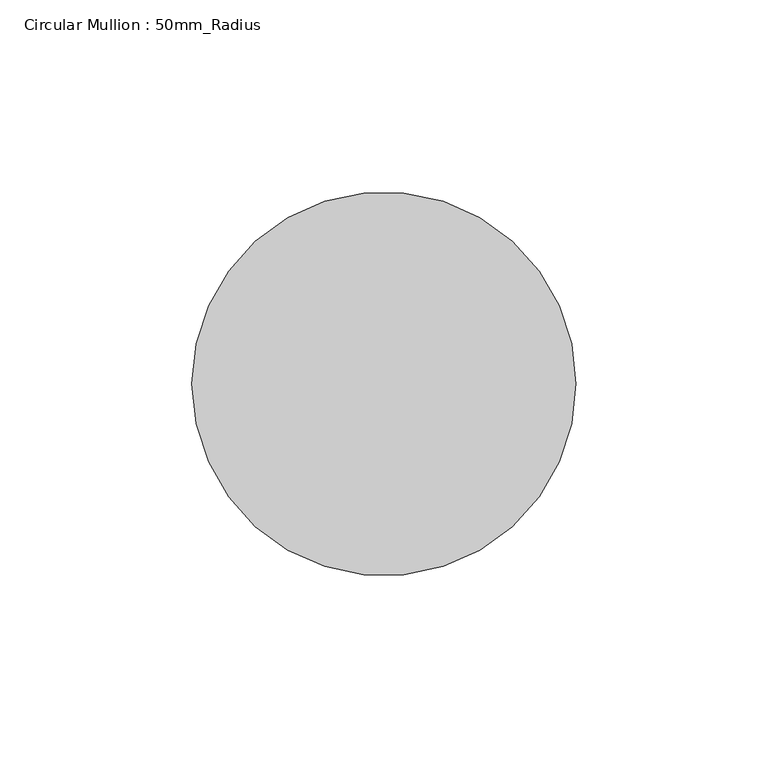
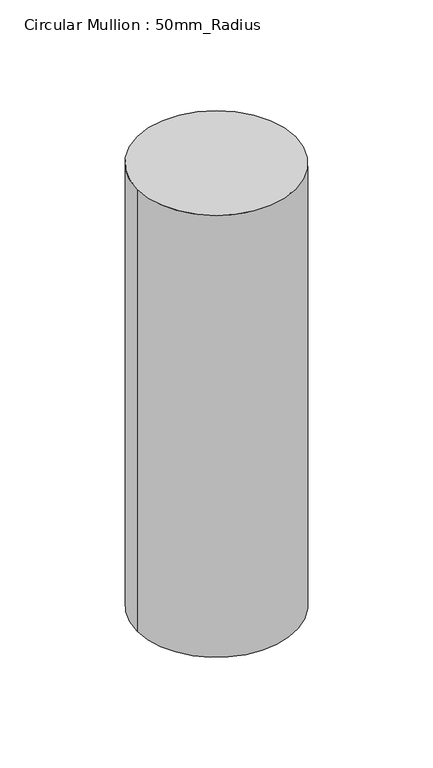
"""IFC4 building model written with IfcOpenShell, lengths in millimetres: member geometry, Circular Mullion : 50mm_Radius."""

from ifc_helpers import new_model, si_unit, point, frame, origin, origin_2d, place, context, project, spatial, circle_curve, trimmed, segment, composite_curve, outline, extrude, source, transform, mapped, element, save


def circular_mullion_50mm_radius_0ba7a25d(model_context):
    return source(origin(), model_context, "Body", "SweptSolid", [
        extrude(outline(composite_curve([segment(trimmed(circle_curve(origin_2d(), 50.0), [point((50.0, 0.0))], [point((-50.0, 0.0))], False, "CARTESIAN"), True, "CONTINUOUS"), segment(trimmed(circle_curve(origin_2d(), 50.0), [point((-50.0, 0.0))], [point((50.0, 0.0))], False, "CARTESIAN"), True, "CONTINUOUS")], self_intersect=False)), frame((0.0, 0.0, -294.9999997), z_axis=(0.0, 0.0, 1.0), x_axis=(1.0, 0.0, 0.0)), (0.0, 0.0, 1.0), 294.9999997),
    ])


if __name__ == "__main__":
    model = new_model("IFC4")
    model_context = context("Model", 3, world=origin())
    ifc_project = project(units=[si_unit("LENGTHUNIT", "METRE", prefix="MILLI")], contexts=[model_context])
    site = spatial("IfcSite", under=ifc_project)
    building = spatial("IfcBuilding", under=site)
    placement = place(None, origin())
    circular_mullion_50mm_radius_shape = circular_mullion_50mm_radius_0ba7a25d(model_context)
    element("IfcMember", 1, ObjectType="Circular Mullion : 50mm_Radius", at=placement, inside=building, context=model_context, shape_type="MappedRepresentation", body=[
        mapped(circular_mullion_50mm_radius_shape, transform((0.0, 0.0, 0.0), x_axis=(1.0, 0.0, 0.0), y_axis=(0.0, 1.0, 0.0), z_axis=(0.0, 0.0, 1.0))),
    ])
    save(model, "model.ifc")

# Revit data of these elements
# Type "Circular Mullion : 50mm_Radius"
#   Keynote = "H11"
#   built-in parameter 1007350 = 0.164042 (stored number, unit not read)
# Element 1 (IfcMember, "Circular Mullion : 50mm_Radius")
#   Materials on its faces: "Aluminium"
# Materials
#   "Aluminium": class "Metal", colour RGB 247 247 247, transparency 0, Description = "Aluminium 6061", Cost = 0
